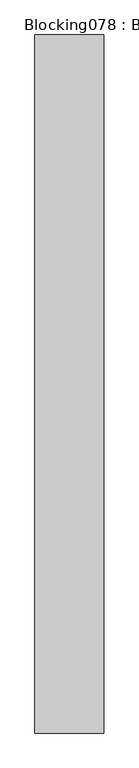
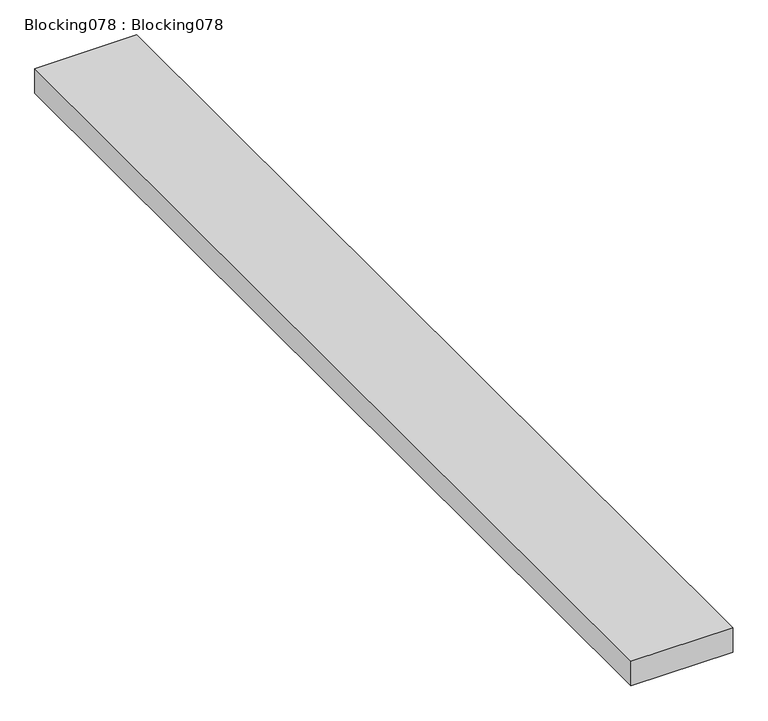
"""IFC4 building model written with IfcOpenShell, lengths in millimetres: proxy geometry, Blocking078 : Blocking078."""

from ifc_helpers import new_model, si_unit, frame, origin, place, context, project, spatial, polyline, outline, extrude, source, transform, mapped, element, save


def blocking078_blocking078_0758a4a0(model_context):
    return source(origin(), model_context, "Body", "SweptSolid", [
        extrude(outline(polyline([(-4797.9038825, -1052.8906574), (-4994.7538825, -1052.8906574), (-4994.7538825, 947.1093426), (-4797.9038825, 947.1093426), (-4797.9038825, -1052.8906574)])), frame((0.0, 0.0, 40131.746), z_axis=(0.0, 0.0, 1.0), x_axis=(1.0, 0.0, 0.0)), (0.0, 0.0, 1.0), 50.8),
    ])


if __name__ == "__main__":
    model = new_model("IFC4")
    model_context = context("Model", 3, world=origin())
    ifc_project = project(units=[si_unit("LENGTHUNIT", "METRE", prefix="MILLI")], contexts=[model_context])
    site = spatial("IfcSite", under=ifc_project)
    building = spatial("IfcBuilding", under=site)
    placement = place(None, origin())
    blocking078_blocking078_shape = blocking078_blocking078_0758a4a0(model_context)
    element("IfcBuildingElementProxy", 1, Name="Blocking078 : Blocking078", ObjectType="Blocking078 : Blocking078", at=placement, inside=building, context=model_context, shape_type="MappedRepresentation", body=[
        mapped(blocking078_blocking078_shape, transform((0.0, 0.0, 0.0), x_axis=(1.0, 0.0, 0.0), y_axis=(0.0, 1.0, 0.0), z_axis=(0.0, 0.0, 1.0))),
    ])
    save(model, "model.ifc")

# Revit data of these elements
# Type "Blocking078 : Blocking078"
#   NameOverride = "Blocking078"
# Element 1 (IfcBuildingElementProxy, "Blocking078 : Blocking078")
#   Materials on its faces: "WOOD BLOCKING AS REQUIRED"
# Materials
#   "WOOD BLOCKING AS REQUIRED": class "Unassigned", colour RGB 166 124 85, transparency 0, Cost = 0
